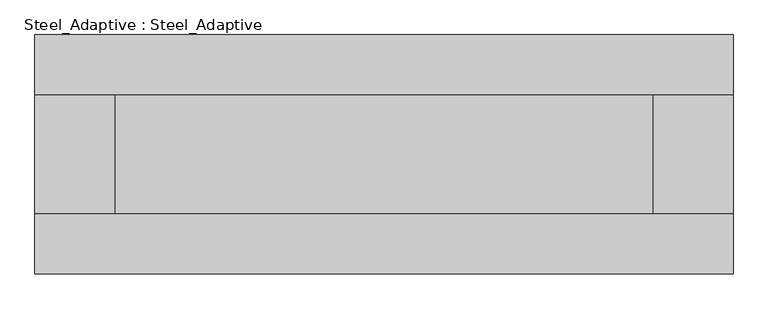
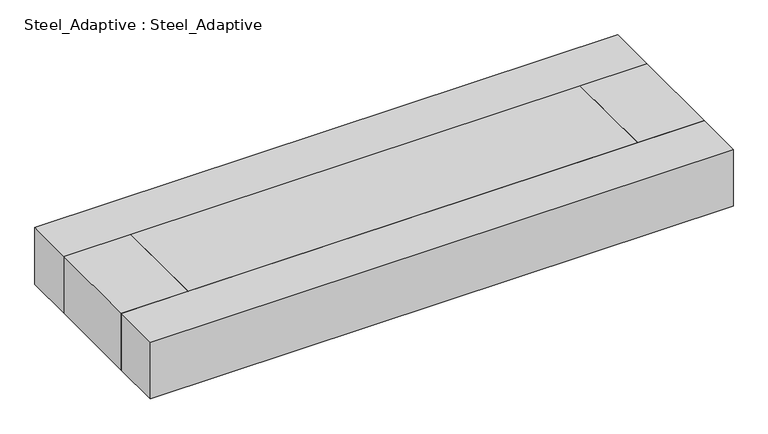
"""IFC4 building model written with IfcOpenShell, lengths in millimetres: proxy geometry, Steel_Adaptive : Steel_Adaptive."""

from ifc_helpers import new_model, si_unit, frame, origin, place, context, project, spatial, polyline, outline, extrude, source, transform, mapped, element, save


def steel_adaptive_steel_adaptive_0ccf134f(model_context):
    return source(origin(), model_context, "Body", "SweptSolid", [
        extrude(outline(polyline([(8750.0, 1500.0), (-8750.0, 1500.0), (-8750.0, 3000.0), (8750.0, 3000.0), (8750.0, 1500.0)])), frame((0.0, 0.0, 55500.0), z_axis=(0.0, 0.0, 1.0), x_axis=(1.0, 0.0, 0.0)), (0.0, 0.0, 1.0), 1800.0),
        extrude(outline(polyline([(-8750.0, -1500.0), (8750.0, -1500.0), (8750.0, -3000.0), (-8750.0, -3000.0), (-8750.0, -1500.0)])), frame((0.0, 0.0, 55500.0), z_axis=(0.0, 0.0, 1.0), x_axis=(1.0, 0.0, 0.0)), (0.0, 0.0, 1.0), 1800.0),
        extrude(outline(polyline([(6750.0, -1500.0), (6750.0, 1500.0), (8750.0, 1500.0), (8750.0, -1500.0), (6750.0, -1500.0)])), frame((0.0, 0.0, 55500.0), z_axis=(0.0, 0.0, 1.0), x_axis=(1.0, 0.0, 0.0)), (0.0, 0.0, 1.0), 1800.0),
        extrude(outline(polyline([(-6750.0, 1500.0), (-6750.0, -1500.0), (-8750.0, -1500.0), (-8750.0, 1500.0), (-6750.0, 1500.0)])), frame((0.0, 0.0, 55500.0), z_axis=(0.0, 0.0, 1.0), x_axis=(1.0, 0.0, 0.0)), (0.0, 0.0, 1.0), 1800.0),
        extrude(outline(polyline([(-6750.0, -1500.0), (-6750.0, 1500.0), (6750.0, 1500.0), (6750.0, -1500.0), (-6750.0, -1500.0)])), frame((0.0, 0.0, 55500.0), z_axis=(0.0, 0.0, 1.0), x_axis=(1.0, 0.0, 0.0)), (0.0, 0.0, 1.0), 1800.0),
    ])


if __name__ == "__main__":
    model = new_model("IFC4")
    model_context = context("Model", 3, world=origin())
    ifc_project = project(units=[si_unit("LENGTHUNIT", "METRE", prefix="MILLI")], contexts=[model_context])
    site = spatial("IfcSite", under=ifc_project)
    building = spatial("IfcBuilding", under=site)
    placement = place(None, origin())
    steel_adaptive_steel_adaptive_shape = steel_adaptive_steel_adaptive_0ccf134f(model_context)
    element("IfcBuildingElementProxy", 1, Name="Steel_Adaptive : Steel_Adaptive", ObjectType="Steel_Adaptive : Steel_Adaptive", at=placement, inside=building, context=model_context, shape_type="MappedRepresentation", body=[
        mapped(steel_adaptive_steel_adaptive_shape, transform((0.0, 0.0, 0.0), x_axis=(1.0, 0.0, 0.0), y_axis=(0.0, 1.0, 0.0), z_axis=(0.0, 0.0, 1.0))),
    ])
    save(model, "model.ifc")

# Revit data of these elements
# Type "Steel_Adaptive : Steel_Adaptive"
#   Width = 3000 mm
#   Top Width = 3000 mm
#   Length = 21000 mm
#   Height [instance default] = 80000 mm
#   Default Elevation = 0
# Element 1 (IfcBuildingElementProxy, "Steel_Adaptive : Steel_Adaptive")
#   Height = 55500 mm
